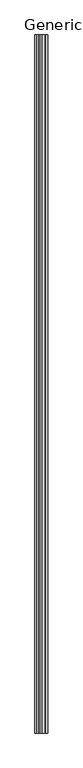
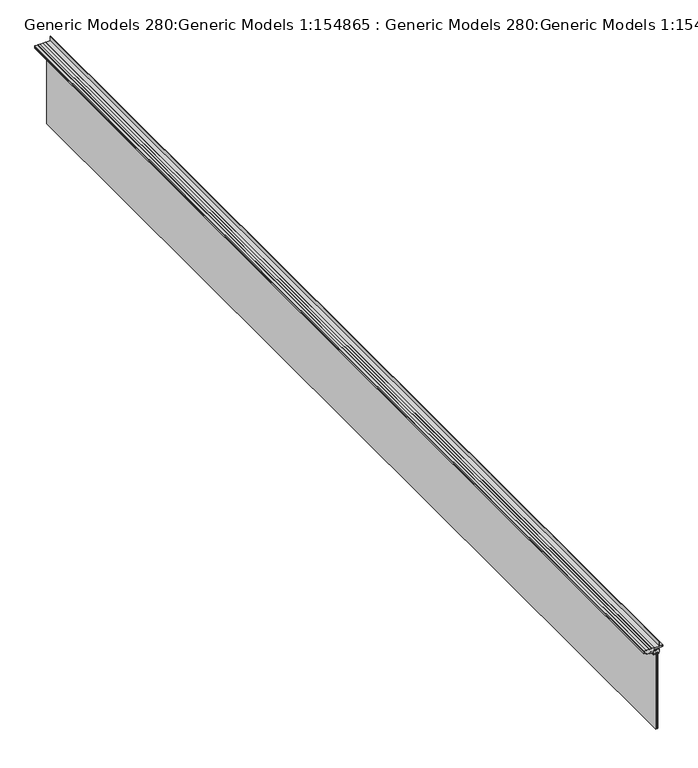
"""IFC4 building model written with IfcOpenShell, lengths in millimetres: proxy geometry, Generic Models 280:Generic Models 1:154865 : Generic Models 280:Generic Models 1:154865."""

from ifc_helpers import new_model, si_unit, point, frame, frame_2d, origin, place, context, project, spatial, polyline, circle_curve, trimmed, segment, composite_curve, outline, extrude, source, transform, mapped, element, save


def generic_models_280_generic_models_1_154865_generic_models_520f1a8e(model_context):
    return source(origin(), model_context, "Body", "SweptSolid", [
        extrude(outline(polyline([(1586.584463, 8383.5218843), (1586.584463, 496.8218843), (1581.821963, 496.8218843), (1581.821963, 8383.5218843), (1586.584463, 8383.5218843)])), frame((0.0, 0.0, 5179.4705773), z_axis=(0.0, 0.0, 1.0), x_axis=(1.0, 0.0, 0.0)), (0.0, 0.0, 1.0), 602.3375481),
        extrude(outline(polyline([(1581.028213, 8383.5218843), (1581.028213, 496.8218843), (1574.679131, 496.8218843), (1574.679131, 8383.5218843), (1581.028213, 8383.5218843)])), frame((0.0, 0.0, 5775.4581253), z_axis=(0.0, 0.0, 1.0), x_axis=(1.0, 0.0, 0.0)), (0.0, 0.0, 1.0), 6.35),
        extrude(outline(composite_curve([segment(polyline([(5779.0212565, 1587.378213), (5777.9981145, 1588.4013551), (5773.7626753, 1588.4013551), (5773.7626753, 1589.537213), (5771.7363015, 1589.537213), (5771.9258518, 1591.9802525), (5779.7316753, 1594.515613), (5779.7316753, 1596.903213), (5802.0328753, 1596.903213)]), True, "CONTINUOUS"), segment(trimmed(circle_curve(frame_2d((5802.0328753, 1594.515613)), 2.3876), [point((5802.0328753, 1596.903213))], [point((5804.4204753, 1594.515613))], False, "CARTESIAN"), True, "CONTINUOUS"), segment(polyline([(5804.4204753, 1594.515613), (5804.4204753, 1591.950213), (5802.3884753, 1591.950213), (5802.3884753, 1590.273813), (5799.0864753, 1590.273813), (5799.0864753, 1588.368813), (5807.0112753, 1588.368813), (5807.0112753, 1582.755413), (5801.7026753, 1582.755413), (5801.7026753, 1570.563413)]), True, "CONTINUOUS"), segment(trimmed(circle_curve(frame_2d((5801.7026753, 1568.582213)), 1.9812), [point((5801.7026753, 1570.563413))], [point((5801.7026753, 1566.601013))], True, "CARTESIAN"), True, "CONTINUOUS"), segment(polyline([(5801.7026753, 1566.601013), (5801.7026753, 1553.266013)]), True, "CONTINUOUS"), segment(trimmed(circle_curve(frame_2d((5800.8898753, 1553.266013)), 0.8128), [point((5801.7026753, 1553.266013))], [point((5800.8898753, 1552.453213))], False, "CARTESIAN"), True, "CONTINUOUS"), segment(polyline([(5800.8898753, 1552.453213), (5782.6018753, 1552.453213), (5782.6018753, 1554.333731), (5781.0009865, 1554.333731), (5781.0009865, 1552.733531), (5773.4571865, 1552.733531), (5773.4571865, 1556.5014505), (5771.2948365, 1556.5014505), (5770.2821865, 1568.329131), (5780.2135865, 1568.329131), (5782.6018753, 1565.9408422), (5782.6018753, 1587.378213), (5779.0212565, 1587.378213)]), True, "CONTINUOUS")], self_intersect=False)), frame((0.0, 496.8218843, 0.0), z_axis=(0.0, 1.0, 0.0), x_axis=(0.0, 0.0, 1.0)), (0.0, 0.0, 1.0), 7886.7),
        extrude(outline(composite_curve([segment(polyline([(5826.8550253, 1498.7668061), (5826.8550253, 1480.6982627), (5818.9048081, 1480.6982627), (5818.9048081, 1488.6484557), (5816.9236306, 1488.6484557), (5816.9236306, 1480.6982627), (5806.9922116, 1480.6982627), (5806.9922116, 1491.0106177), (5806.179422, 1491.7980696), (5806.179422, 1494.9730696), (5802.2170185, 1494.9730696), (5802.2170185, 1496.5732627), (5799.0420185, 1500.5102316), (5799.0420185, 1502.1104247), (5796.654422, 1502.1104247), (5796.654422, 1521.1604247), (5790.3225895, 1521.1604247), (5790.3225895, 1550.5736487), (5793.4975895, 1550.5736487), (5793.4975895, 1547.5256758), (5802.1843895, 1547.5256758), (5802.1843895, 1529.9996758), (5804.4703895, 1529.9996758), (5804.4703895, 1547.5256758), (5805.410186, 1547.5256758), (5805.410186, 1555.9330115), (5813.3603791, 1555.9330115), (5813.3603791, 1557.9142859), (5806.9414395, 1557.9142859), (5806.9414395, 1561.927413), (5811.8182321, 1561.927413), (5811.8182321, 1596.877813), (5814.240602, 1624.741613), (5823.1720253, 1624.741613), (5823.1720253, 1616.8380474), (5825.4580253, 1616.8380474), (5825.4580253, 1623.1880474), (5826.8550253, 1623.1880474), (5826.8550253, 1598.300213), (5862.2221123, 1598.300213)]), True, "CONTINUOUS"), segment(trimmed(circle_curve(frame_2d((5862.224572, 1597.6017132)), 0.6985041), [point((5862.2221123, 1598.300213))], [point((5862.2269129, 1596.903213))], False, "CARTESIAN"), True, "CONTINUOUS"), segment(polyline([(5862.2269129, 1596.903213), (5826.8550253, 1596.903213), (5826.8550253, 1560.4340452), (5823.6800253, 1560.4340452), (5823.6800253, 1558.1480452), (5826.8550253, 1558.1480452), (5826.8550253, 1541.0486627), (5824.7722253, 1541.0486627), (5824.7722253, 1537.8736627), (5826.8550253, 1537.8736627), (5826.8550253, 1520.846563), (5823.6800253, 1520.846563), (5823.6800253, 1518.5605591), (5826.8550253, 1518.5605591), (5826.8550253, 1501.05281), (5823.6800253, 1501.05281), (5823.6800253, 1498.7668061), (5826.8550253, 1498.7668061)]), True, "CONTINUOUS")], self_intersect=False)), frame((0.0, 496.8218843, 0.0), z_axis=(0.0, 1.0, 0.0), x_axis=(0.0, 0.0, 1.0)), (0.0, 0.0, 1.0), 7886.7),
        extrude(outline(polyline([(1573.885381, 8383.5218843), (1573.885381, 496.8218843), (1569.122881, 496.8218843), (1569.122881, 8383.5218843), (1573.885381, 8383.5218843)])), frame((0.0, 0.0, 5179.4705773), z_axis=(0.0, 0.0, 1.0), x_axis=(1.0, 0.0, 0.0)), (0.0, 0.0, 1.0), 602.3375481),
    ])


if __name__ == "__main__":
    model = new_model("IFC4")
    model_context = context("Model", 3, world=origin())
    ifc_project = project(units=[si_unit("LENGTHUNIT", "METRE", prefix="MILLI")], contexts=[model_context])
    site = spatial("IfcSite", under=ifc_project)
    building = spatial("IfcBuilding", under=site)
    placement = place(None, origin())
    generic_models_280_generic_models_1_154865_generic_models_shape = generic_models_280_generic_models_1_154865_generic_models_520f1a8e(model_context)
    element("IfcBuildingElementProxy", 1, Name="Generic Models 280:Generic Models 1:154865 : Generic Models 280:Generic Models 1:154865", ObjectType="Generic Models 280:Generic Models 1:154865 : Generic Models 280:Generic Models 1:154865", at=placement, inside=building, context=model_context, shape_type="MappedRepresentation", body=[
        mapped(generic_models_280_generic_models_1_154865_generic_models_shape, transform((0.0, 0.0, 0.0), x_axis=(1.0, 0.0, 0.0), y_axis=(0.0, 1.0, 0.0), z_axis=(0.0, 0.0, 1.0))),
    ])
    save(model, "model.ifc")

# Revit data of these elements
# Type "Generic Models 280:Generic Models 1:154865 : Generic Models 280:Generic Models 1:154865"
#   NameOverride = "Generic Models 280:Generic Models 1:154865"
#   ObjectTypeOverride = "Generic Models 280:Generic Models 1"
#   Reference = "Generic Models 1"
#   Category = "Generic Models"
#   Tag = "154865"
# Element 1 (IfcBuildingElementProxy, "Generic Models 280:Generic Models 1:154865 : Generic Models 280:Generic Models 1:154865")
#   Materials on its faces: "_WINDOW PER SCHEDULE 24593"
# Materials
#   "_WINDOW PER SCHEDULE 24593": class "Unassigned", colour RGB 255 255 255, transparency 0
